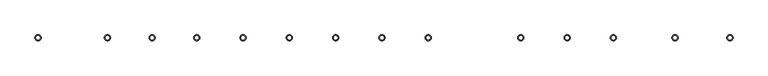
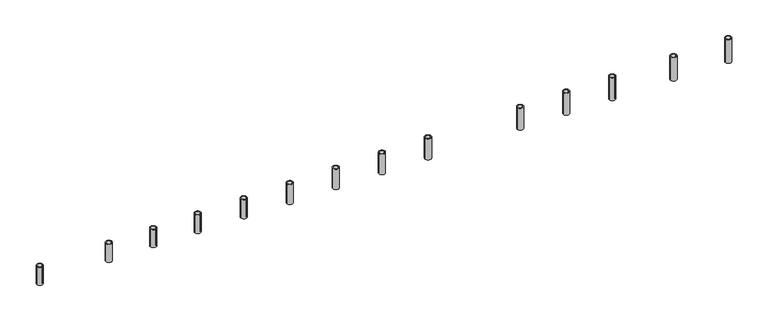
"""IFC4 building model written with IfcOpenShell, lengths in millimetres: column geometry, Column Encasement : Column Encasement."""

from ifc_helpers import new_model, si_unit, point, frame, frame_2d, origin, origin_2d, place, context, project, spatial, circle_curve, trimmed, segment, composite_curve, outline, extrude, source, transform, mapped, element, save


def column_0b6fd7b6(model_context):
    return source(origin(), model_context, "Body", "SweptSolid", [
        extrude(outline(composite_curve([segment(trimmed(circle_curve(frame_2d((-85039.2, 0.0)), 381.0), [point((-85420.2, 0.0))], [point((-84658.2, 0.0))], False, "CARTESIAN"), True, "CONTINUOUS"), segment(trimmed(circle_curve(frame_2d((-85039.2, 0.0)), 381.0), [point((-84658.2, 0.0))], [point((-85420.2, 0.0))], False, "CARTESIAN"), True, "CONTINUOUS")], self_intersect=False), holes=[composite_curve([segment(trimmed(circle_curve(frame_2d((-85039.2, 0.0)), 254.0), [point((-85293.2, 0.0))], [point((-84785.2, 0.0))], True, "CARTESIAN"), True, "CONTINUOUS"), segment(trimmed(circle_curve(frame_2d((-85039.2, 0.0)), 254.0), [point((-84785.2, 0.0))], [point((-85293.2, 0.0))], True, "CARTESIAN"), True, "CONTINUOUS")], self_intersect=False)]), frame((0.0, 0.0, 13064.5726821), z_axis=(0.0, 0.0, 1.0), x_axis=(1.0, 0.0, 0.0)), (0.0, 0.0, 1.0), 2346.8773179),
        extrude(outline(composite_curve([segment(trimmed(circle_curve(frame_2d((-76504.8, 0.0)), 381.0), [point((-76885.8, 0.0))], [point((-76123.8, 0.0))], False, "CARTESIAN"), True, "CONTINUOUS"), segment(trimmed(circle_curve(frame_2d((-76504.8, 0.0)), 381.0), [point((-76123.8, 0.0))], [point((-76885.8, 0.0))], False, "CARTESIAN"), True, "CONTINUOUS")], self_intersect=False), holes=[composite_curve([segment(trimmed(circle_curve(frame_2d((-76504.8, 0.0)), 254.0), [point((-76758.8, 0.0))], [point((-76250.8, 0.0))], True, "CARTESIAN"), True, "CONTINUOUS"), segment(trimmed(circle_curve(frame_2d((-76504.8, 0.0)), 254.0), [point((-76250.8, 0.0))], [point((-76758.8, 0.0))], True, "CARTESIAN"), True, "CONTINUOUS")], self_intersect=False)]), frame((0.0, 0.0, 13065.4051519), z_axis=(0.0, 0.0, 1.0), x_axis=(1.0, 0.0, 0.0)), (0.0, 0.0, 1.0), 2346.0448481),
        extrude(outline(composite_curve([segment(trimmed(circle_curve(frame_2d((-71018.4, 0.0)), 381.0), [point((-71399.4, 0.0))], [point((-70637.4, 0.0))], False, "CARTESIAN"), True, "CONTINUOUS"), segment(trimmed(circle_curve(frame_2d((-71018.4, 0.0)), 381.0), [point((-70637.4, 0.0))], [point((-71399.4, 0.0))], False, "CARTESIAN"), True, "CONTINUOUS")], self_intersect=False), holes=[composite_curve([segment(trimmed(circle_curve(frame_2d((-71018.4, 0.0)), 254.0), [point((-71272.4, 0.0))], [point((-70764.4, 0.0))], True, "CARTESIAN"), True, "CONTINUOUS"), segment(trimmed(circle_curve(frame_2d((-71018.4, 0.0)), 254.0), [point((-70764.4, 0.0))], [point((-71272.4, 0.0))], True, "CARTESIAN"), True, "CONTINUOUS")], self_intersect=False)]), frame((0.0, 0.0, 13087.85604), z_axis=(0.0, 0.0, 1.0), x_axis=(1.0, 0.0, 0.0)), (0.0, 0.0, 1.0), 2323.59396),
        extrude(outline(composite_curve([segment(trimmed(circle_curve(frame_2d((-65532.0, 0.0)), 381.0), [point((-65913.0, 0.0))], [point((-65151.0, 0.0))], False, "CARTESIAN"), True, "CONTINUOUS"), segment(trimmed(circle_curve(frame_2d((-65532.0, 0.0)), 381.0), [point((-65151.0, 0.0))], [point((-65913.0, 0.0))], False, "CARTESIAN"), True, "CONTINUOUS")], self_intersect=False), holes=[composite_curve([segment(trimmed(circle_curve(frame_2d((-65532.0, 0.0)), 254.0), [point((-65786.0, 0.0))], [point((-65278.0, 0.0))], True, "CARTESIAN"), True, "CONTINUOUS"), segment(trimmed(circle_curve(frame_2d((-65532.0, 0.0)), 254.0), [point((-65278.0, 0.0))], [point((-65786.0, 0.0))], True, "CARTESIAN"), True, "CONTINUOUS")], self_intersect=False)]), frame((0.0, 0.0, 12999.9023766), z_axis=(0.0, 0.0, 1.0), x_axis=(1.0, 0.0, 0.0)), (0.0, 0.0, 1.0), 2411.5476234),
        extrude(outline(composite_curve([segment(trimmed(circle_curve(frame_2d((-59842.4, 0.0)), 381.0), [point((-60223.4, 0.0))], [point((-59461.4, 0.0))], False, "CARTESIAN"), True, "CONTINUOUS"), segment(trimmed(circle_curve(frame_2d((-59842.4, 0.0)), 381.0), [point((-59461.4, 0.0))], [point((-60223.4, 0.0))], False, "CARTESIAN"), True, "CONTINUOUS")], self_intersect=False), holes=[composite_curve([segment(trimmed(circle_curve(frame_2d((-59842.4, 0.0)), 254.0), [point((-60096.4, 0.0))], [point((-59588.4, 0.0))], True, "CARTESIAN"), True, "CONTINUOUS"), segment(trimmed(circle_curve(frame_2d((-59842.4, 0.0)), 254.0), [point((-59588.4, 0.0))], [point((-60096.4, 0.0))], True, "CARTESIAN"), True, "CONTINUOUS")], self_intersect=False)]), frame((0.0, 0.0, 12946.9818447), z_axis=(0.0, 0.0, 1.0), x_axis=(1.0, 0.0, 0.0)), (0.0, 0.0, 1.0), 2464.4681553),
        extrude(outline(composite_curve([segment(trimmed(circle_curve(frame_2d((-54152.8, 0.0)), 381.0), [point((-54533.8, 0.0))], [point((-53771.8, 0.0))], False, "CARTESIAN"), True, "CONTINUOUS"), segment(trimmed(circle_curve(frame_2d((-54152.8, 0.0)), 381.0), [point((-53771.8, 0.0))], [point((-54533.8, 0.0))], False, "CARTESIAN"), True, "CONTINUOUS")], self_intersect=False), holes=[composite_curve([segment(trimmed(circle_curve(frame_2d((-54152.8, 0.0)), 254.0), [point((-54406.8, 0.0))], [point((-53898.8, 0.0))], True, "CARTESIAN"), True, "CONTINUOUS"), segment(trimmed(circle_curve(frame_2d((-54152.8, 0.0)), 254.0), [point((-53898.8, 0.0))], [point((-54406.8, 0.0))], True, "CARTESIAN"), True, "CONTINUOUS")], self_intersect=False)]), frame((0.0, 0.0, 12824.2377413), z_axis=(0.0, 0.0, 1.0), x_axis=(1.0, 0.0, 0.0)), (0.0, 0.0, 1.0), 2587.2122587),
        extrude(outline(composite_curve([segment(trimmed(circle_curve(frame_2d((-48463.2, 0.0)), 381.0), [point((-48844.2, 0.0))], [point((-48082.2, 0.0))], False, "CARTESIAN"), True, "CONTINUOUS"), segment(trimmed(circle_curve(frame_2d((-48463.2, 0.0)), 381.0), [point((-48082.2, 0.0))], [point((-48844.2, 0.0))], False, "CARTESIAN"), True, "CONTINUOUS")], self_intersect=False), holes=[composite_curve([segment(trimmed(circle_curve(frame_2d((-48463.2, 0.0)), 254.0), [point((-48717.2, 0.0))], [point((-48209.2, 0.0))], True, "CARTESIAN"), True, "CONTINUOUS"), segment(trimmed(circle_curve(frame_2d((-48463.2, 0.0)), 254.0), [point((-48209.2, 0.0))], [point((-48717.2, 0.0))], True, "CARTESIAN"), True, "CONTINUOUS")], self_intersect=False)]), frame((0.0, 0.0, 12771.8660567), z_axis=(0.0, 0.0, 1.0), x_axis=(1.0, 0.0, 0.0)), (0.0, 0.0, 1.0), 2639.5839433),
        extrude(outline(composite_curve([segment(trimmed(circle_curve(frame_2d((-42773.6, 0.0)), 381.0), [point((-43154.6, 0.0))], [point((-42392.6, 0.0))], False, "CARTESIAN"), True, "CONTINUOUS"), segment(trimmed(circle_curve(frame_2d((-42773.6, 0.0)), 381.0), [point((-42392.6, 0.0))], [point((-43154.6, 0.0))], False, "CARTESIAN"), True, "CONTINUOUS")], self_intersect=False), holes=[composite_curve([segment(trimmed(circle_curve(frame_2d((-42773.6, 0.0)), 254.0), [point((-43027.6, 0.0))], [point((-42519.6, 0.0))], True, "CARTESIAN"), True, "CONTINUOUS"), segment(trimmed(circle_curve(frame_2d((-42773.6, 0.0)), 254.0), [point((-42519.6, 0.0))], [point((-43027.6, 0.0))], True, "CARTESIAN"), True, "CONTINUOUS")], self_intersect=False)]), frame((0.0, 0.0, 12736.16224), z_axis=(0.0, 0.0, 1.0), x_axis=(1.0, 0.0, 0.0)), (0.0, 0.0, 1.0), 2675.28776),
        extrude(outline(composite_curve([segment(trimmed(circle_curve(frame_2d((-37084.0, 0.0)), 381.0), [point((-37465.0, 0.0))], [point((-36703.0, 0.0))], False, "CARTESIAN"), True, "CONTINUOUS"), segment(trimmed(circle_curve(frame_2d((-37084.0, 0.0)), 381.0), [point((-36703.0, 0.0))], [point((-37465.0, 0.0))], False, "CARTESIAN"), True, "CONTINUOUS")], self_intersect=False), holes=[composite_curve([segment(trimmed(circle_curve(frame_2d((-37084.0, 0.0)), 254.0), [point((-37338.0, 0.0))], [point((-36830.0, 0.0))], True, "CARTESIAN"), True, "CONTINUOUS"), segment(trimmed(circle_curve(frame_2d((-37084.0, 0.0)), 254.0), [point((-36830.0, 0.0))], [point((-37338.0, 0.0))], True, "CARTESIAN"), True, "CONTINUOUS")], self_intersect=False)]), frame((0.0, 0.0, 12681.2581379), z_axis=(0.0, 0.0, 1.0), x_axis=(1.0, 0.0, 0.0)), (0.0, 0.0, 1.0), 2730.1918621),
        extrude(outline(composite_curve([segment(trimmed(circle_curve(frame_2d((-25704.8, 0.0)), 381.0), [point((-26085.8, 0.0))], [point((-25323.8, 0.0))], False, "CARTESIAN"), True, "CONTINUOUS"), segment(trimmed(circle_curve(frame_2d((-25704.8, 0.0)), 381.0), [point((-25323.8, 0.0))], [point((-26085.8, 0.0))], False, "CARTESIAN"), True, "CONTINUOUS")], self_intersect=False), holes=[composite_curve([segment(trimmed(circle_curve(frame_2d((-25704.8, 0.0)), 254.0), [point((-25958.8, 0.0))], [point((-25450.8, 0.0))], True, "CARTESIAN"), True, "CONTINUOUS"), segment(trimmed(circle_curve(frame_2d((-25704.8, 0.0)), 254.0), [point((-25450.8, 0.0))], [point((-25958.8, 0.0))], True, "CARTESIAN"), True, "CONTINUOUS")], self_intersect=False)]), frame((0.0, 0.0, 12599.813627), z_axis=(0.0, 0.0, 1.0), x_axis=(1.0, 0.0, 0.0)), (0.0, 0.0, 1.0), 2811.636373),
        extrude(outline(composite_curve([segment(trimmed(circle_curve(frame_2d((-20015.2, 0.0)), 381.0), [point((-20396.2, 0.0))], [point((-19634.2, 0.0))], False, "CARTESIAN"), True, "CONTINUOUS"), segment(trimmed(circle_curve(frame_2d((-20015.2, 0.0)), 381.0), [point((-19634.2, 0.0))], [point((-20396.2, 0.0))], False, "CARTESIAN"), True, "CONTINUOUS")], self_intersect=False), holes=[composite_curve([segment(trimmed(circle_curve(frame_2d((-20015.2, 0.0)), 254.0), [point((-20269.2, 0.0))], [point((-19761.2, 0.0))], True, "CARTESIAN"), True, "CONTINUOUS"), segment(trimmed(circle_curve(frame_2d((-20015.2, 0.0)), 254.0), [point((-19761.2, 0.0))], [point((-20269.2, 0.0))], True, "CARTESIAN"), True, "CONTINUOUS")], self_intersect=False)]), frame((0.0, 0.0, 12539.4776195), z_axis=(0.0, 0.0, 1.0), x_axis=(1.0, 0.0, 0.0)), (0.0, 0.0, 1.0), 2871.9723806),
        extrude(outline(composite_curve([segment(trimmed(circle_curve(frame_2d((-14325.6, 0.0)), 381.0), [point((-14706.6, 0.0))], [point((-13944.6, 0.0))], False, "CARTESIAN"), True, "CONTINUOUS"), segment(trimmed(circle_curve(frame_2d((-14325.6, 0.0)), 381.0), [point((-13944.6, 0.0))], [point((-14706.6, 0.0))], False, "CARTESIAN"), True, "CONTINUOUS")], self_intersect=False), holes=[composite_curve([segment(trimmed(circle_curve(frame_2d((-14325.6, 0.0)), 254.0), [point((-14579.6, 0.0))], [point((-14071.6, 0.0))], True, "CARTESIAN"), True, "CONTINUOUS"), segment(trimmed(circle_curve(frame_2d((-14325.6, 0.0)), 254.0), [point((-14071.6, 0.0))], [point((-14579.6, 0.0))], True, "CARTESIAN"), True, "CONTINUOUS")], self_intersect=False)]), frame((0.0, 0.0, 12462.2655781), z_axis=(0.0, 0.0, 1.0), x_axis=(1.0, 0.0, 0.0)), (0.0, 0.0, 1.0), 2949.1844219),
        extrude(outline(composite_curve([segment(trimmed(circle_curve(frame_2d((-6756.4, 0.0)), 381.0), [point((-7137.4, 0.0))], [point((-6375.4, 0.0))], False, "CARTESIAN"), True, "CONTINUOUS"), segment(trimmed(circle_curve(frame_2d((-6756.4, 0.0)), 381.0), [point((-6375.4, 0.0))], [point((-7137.4, 0.0))], False, "CARTESIAN"), True, "CONTINUOUS")], self_intersect=False), holes=[composite_curve([segment(trimmed(circle_curve(frame_2d((-6756.4, 0.0)), 254.0), [point((-7010.4, 0.0))], [point((-6502.4, 0.0))], True, "CARTESIAN"), True, "CONTINUOUS"), segment(trimmed(circle_curve(frame_2d((-6756.4, 0.0)), 254.0), [point((-6502.4, 0.0))], [point((-7010.4, 0.0))], True, "CARTESIAN"), True, "CONTINUOUS")], self_intersect=False)]), frame((0.0, 0.0, 12372.7089215), z_axis=(0.0, 0.0, 1.0), x_axis=(1.0, 0.0, 0.0)), (0.0, 0.0, 1.0), 3038.7410785),
        extrude(outline(composite_curve([segment(trimmed(circle_curve(origin_2d(), 381.0), [point((-381.0, 0.0))], [point((381.0, 0.0))], False, "CARTESIAN"), True, "CONTINUOUS"), segment(trimmed(circle_curve(origin_2d(), 381.0), [point((381.0, 0.0))], [point((-381.0, 0.0))], False, "CARTESIAN"), True, "CONTINUOUS")], self_intersect=False), holes=[composite_curve([segment(trimmed(circle_curve(origin_2d(), 254.0), [point((-254.0, 0.0))], [point((254.0, 0.0))], True, "CARTESIAN"), True, "CONTINUOUS"), segment(trimmed(circle_curve(origin_2d(), 254.0), [point((254.0, 0.0))], [point((-254.0, 0.0))], True, "CARTESIAN"), True, "CONTINUOUS")], self_intersect=False)]), frame((0.0, 0.0, 12317.4125), z_axis=(0.0, 0.0, 1.0), x_axis=(1.0, 0.0, 0.0)), (0.0, 0.0, 1.0), 3094.0375),
    ])


if __name__ == "__main__":
    model = new_model("IFC4")
    model_context = context("Model", 3, world=origin())
    ifc_project = project(units=[si_unit("LENGTHUNIT", "METRE", prefix="MILLI")], contexts=[model_context])
    site = spatial("IfcSite", under=ifc_project)
    building = spatial("IfcBuilding", under=site)
    placement = place(None, origin())
    column_shape = column_0b6fd7b6(model_context)
    element("IfcColumn", 1, ObjectType="Column Encasement : Column Encasement", at=placement, inside=building, context=model_context, shape_type="MappedRepresentation", body=[
        mapped(column_shape, transform((0.0, 0.0, 0.0), x_axis=(1.0, 0.0, 0.0), y_axis=(0.0, 1.0, 0.0), z_axis=(0.0, 0.0, 1.0))),
    ])
    save(model, "model.ifc")

# Revit data of these elements
# Element 1 (IfcColumn, "Column Encasement : Column Encasement")
#   Materials on its faces: "05 - Metal - Aluminum"
# Materials
#   "05 - Metal - Aluminum": class "Unassigned", colour RGB 247 247 247, transparency 0, Description = "Aluminum"
